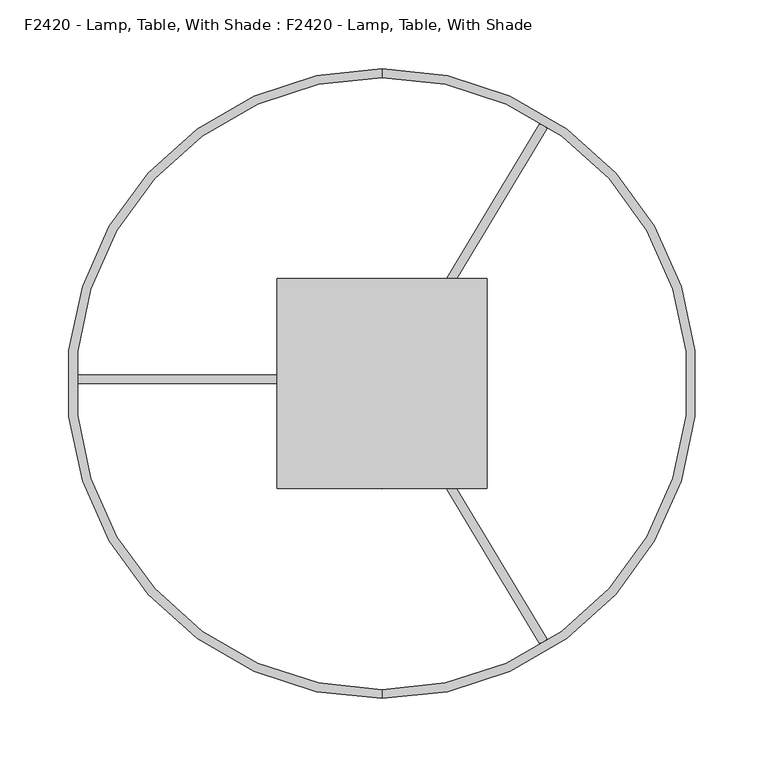
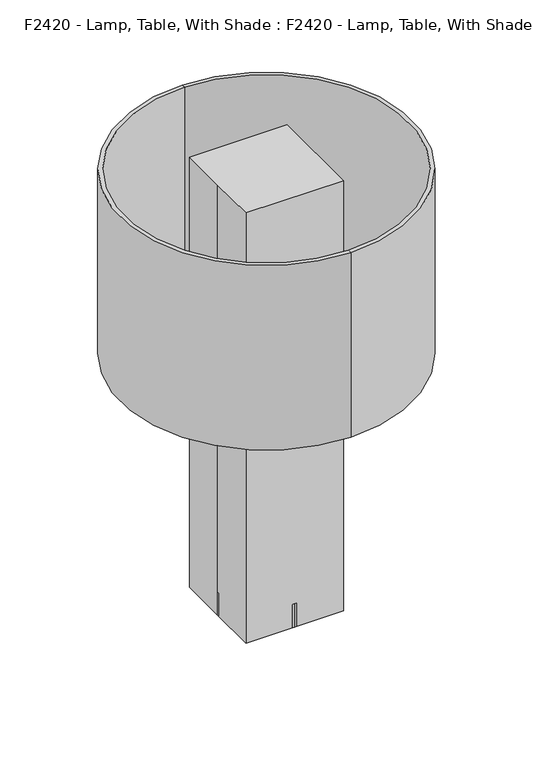
"""IFC4 building model written with IfcOpenShell, lengths in millimetres: proxy geometry, F2420 - Lamp, Table, With Shade : F2420 - Lamp, Table, With Shade."""

import ifcopenshell
import ifcopenshell.guid

model = None  # the IFC model being written
_history = None  # IfcOwnerHistory: only IFC2X3 demands one
_inside = {}  # id of a spatial element -> (the spatial element, [elements in it])
_under = {}  # id of a project, library or spatial element -> (it, [spatial elements below it])
_declared = {}  # id of a project -> (the project, [libraries it declares])
_typed = {}  # id of a type object -> (the type object, [elements of that type])
_made_of = {}  # id of a material, layer set ... -> (it, [elements and type objects made of it])


def new_model(schema):
    """Start an empty IFC model of exactly this schema.

    Asked for "IFC4X3", IfcOpenShell would pick the latest addendum, in which some entities
    have other attributes; the version numbers below select the first issue.
    IFC2X3 requires an IfcOwnerHistory on every rooted entity: one is made here for all.
    """
    global model, _history
    if schema == "IFC4X3":
        model = ifcopenshell.file(schema_version=(4, 3, 0, 0))
    else:
        model = ifcopenshell.file(schema=schema)
    _inside.clear()
    _under.clear()
    _declared.clear()
    _typed.clear()
    _made_of.clear()
    _history = None
    if model.schema == "IFC2X3":
        org = make("IfcOrganization", Name="unknown")
        user = make(
            "IfcPersonAndOrganization",
            ThePerson=make("IfcPerson", FamilyName="unknown"),
            TheOrganization=org,
        )
        app = make(
            "IfcApplication",
            ApplicationDeveloper=org,
            Version="unknown",
            ApplicationFullName="unknown",
            ApplicationIdentifier="unknown",
        )
        _history = make(
            "IfcOwnerHistory",
            OwningUser=user,
            OwningApplication=app,
            ChangeAction="ADDED",
            CreationDate=0,
        )
    return model


def make(cls, **values):
    """One entity of the class cls with the attributes given. An attribute that is None is left unset."""
    return model.create_entity(
        cls, **{name: value for name, value in values.items() if value is not None}
    )


def rooted(cls, **values):
    """An entity with a GlobalId (a new one), such as an element, a storey or a relation."""
    return make(cls, GlobalId=ifcopenshell.guid.new(), OwnerHistory=_history, **values)


def si_unit(unit_type, name, prefix=None):
    """IfcSIUnit, for example si_unit("LENGTHUNIT", "METRE", prefix="MILLI")."""
    return make("IfcSIUnit", UnitType=unit_type, Prefix=prefix, Name=name)


def assignment(units):
    """IfcUnitAssignment: the units of a project."""
    return None if units is None else make("IfcUnitAssignment", Units=units)


def point(xyz):
    """IfcCartesianPoint."""
    return None if xyz is None else make("IfcCartesianPoint", Coordinates=xyz)


def direction(xyz):
    """IfcDirection."""
    return None if xyz is None else make("IfcDirection", DirectionRatios=xyz)


def frame(location, z_axis=None, x_axis=None):
    """IfcAxis2Placement3D, a coordinate frame: its origin and axes. An axis left out is left unset."""
    return make(
        "IfcAxis2Placement3D",
        Location=point(location),
        Axis=direction(z_axis),
        RefDirection=direction(x_axis),
    )


def frame_2d(location, x_axis=None):
    """IfcAxis2Placement2D, a coordinate frame in the plane: its origin and x axis."""
    return make(
        "IfcAxis2Placement2D", Location=point(location), RefDirection=direction(x_axis)
    )


def origin():
    """The frame at (0, 0, 0) with its axes left unset."""
    return frame((0.0, 0.0, 0.0))


def origin_with_axes():
    """The frame at (0, 0, 0) with the z axis (0, 0, 1) and the x axis (1, 0, 0) written out."""
    return frame((0.0, 0.0, 0.0), z_axis=(0.0, 0.0, 1.0), x_axis=(1.0, 0.0, 0.0))


def place(relative_to, where):
    """IfcLocalPlacement: puts the frame where relative to a parent placement (None: the world)."""
    return make(
        "IfcLocalPlacement", PlacementRelTo=relative_to, RelativePlacement=where
    )


def context(
    kind, dimensions, precision=None, world=None, true_north=None, identifier=None
):
    """IfcGeometricRepresentationContext, for example the 3D "Model" context."""
    return make(
        "IfcGeometricRepresentationContext",
        ContextIdentifier=identifier,
        ContextType=kind,
        CoordinateSpaceDimension=dimensions,
        Precision=precision,
        WorldCoordinateSystem=world,
        TrueNorth=true_north,
    )


def project(units=None, contexts=None):
    """IfcProject with its units and contexts."""
    return rooted(
        "IfcProject",
        Name="project",
        RepresentationContexts=contexts,
        UnitsInContext=assignment(units),
    )


def spatial(cls, under=None, at=None, **own):
    """A site, building, storey or space (cls), placed at a placement, below another one or the project."""
    s = rooted(cls, ObjectPlacement=at, **own)
    if under is not None:
        _under.setdefault(under.id(), (under, []))[1].append(s)
    return s


def polyline(points):
    """IfcPolyline through the points."""
    return make("IfcPolyline", Points=[point(p) for p in points])


def circle_curve(where, radius):
    """IfcCircle in the frame where."""
    return make("IfcCircle", Position=where, Radius=radius)


def ellipse_curve(where, semi_axis1, semi_axis2):
    """IfcEllipse in the frame where."""
    return make(
        "IfcEllipse", Position=where, SemiAxis1=semi_axis1, SemiAxis2=semi_axis2
    )


def trimmed(basis, trim1, trim2, sense, master):
    """IfcTrimmedCurve: the piece of a basis curve between two trims."""
    return make(
        "IfcTrimmedCurve",
        BasisCurve=basis,
        Trim1=trim1,
        Trim2=trim2,
        SenseAgreement=sense,
        MasterRepresentation=master,
    )


def segment(curve, same_sense, transition):
    """IfcCompositeCurveSegment."""
    return make(
        "IfcCompositeCurveSegment",
        Transition=transition,
        SameSense=same_sense,
        ParentCurve=curve,
    )


def composite_curve(segments, self_intersect=None):
    """IfcCompositeCurve: segments joined end to end."""
    return make("IfcCompositeCurve", Segments=segments, SelfIntersect=self_intersect)


def outline(outer, holes=None, kind="AREA"):
    """IfcArbitraryClosedProfileDef: a profile drawn as a closed curve; with holes, ...WithVoids."""
    if holes is None:
        return make("IfcArbitraryClosedProfileDef", ProfileType=kind, OuterCurve=outer)
    return make(
        "IfcArbitraryProfileDefWithVoids",
        ProfileType=kind,
        OuterCurve=outer,
        InnerCurves=holes,
    )


def extrude(swept, where, along, depth):
    """IfcExtrudedAreaSolid: the profile swept, set in the frame where, extruded along a direction by depth."""
    return make(
        "IfcExtrudedAreaSolid",
        SweptArea=swept,
        Position=where,
        ExtrudedDirection=direction(along),
        Depth=depth,
    )


def shape(context_of_items, identifier, shape_type, items):
    """IfcShapeRepresentation: the items that make up one representation, for example the "Body"."""
    return make(
        "IfcShapeRepresentation",
        ContextOfItems=context_of_items,
        RepresentationIdentifier=identifier,
        RepresentationType=shape_type,
        Items=items,
    )


def source(mapping_origin, context_of_items, identifier, shape_type, items):
    """IfcRepresentationMap: a shape defined once, which mapped items show again and again."""
    return make(
        "IfcRepresentationMap",
        MappingOrigin=mapping_origin,
        MappedRepresentation=shape(context_of_items, identifier, shape_type, items),
    )


def transform(
    local_origin,
    x_axis=None,
    y_axis=None,
    z_axis=None,
    scale=None,
    scale2=None,
    scale3=None,
    uniform=True,
):
    """IfcCartesianTransformationOperator3D, or its non-uniform kind. x_axis, y_axis, z_axis: its Axis1, 2, 3."""
    if uniform:
        return make(
            "IfcCartesianTransformationOperator3D",
            Axis1=direction(x_axis),
            Axis2=direction(y_axis),
            LocalOrigin=point(local_origin),
            Scale=scale,
            Axis3=direction(z_axis),
        )
    return make(
        "IfcCartesianTransformationOperator3DnonUniform",
        Axis1=direction(x_axis),
        Axis2=direction(y_axis),
        LocalOrigin=point(local_origin),
        Scale=scale,
        Axis3=direction(z_axis),
        Scale2=scale2,
        Scale3=scale3,
    )


def mapped(mapping_source, mapping_target):
    """IfcMappedItem: shows the shape of a source again, moved by a transform."""
    return make(
        "IfcMappedItem", MappingSource=mapping_source, MappingTarget=mapping_target
    )


def made_of(thing, what):
    """Note that an element or type object is made of a material, layer set ...; save() writes the relation."""
    if what is not None:
        _made_of.setdefault(what.id(), (what, []))[1].append(thing)
    return thing


def element(
    cls,
    number,
    at=None,
    inside=None,
    cuts=None,
    type_object=None,
    material=None,
    context=None,
    identifier="Body",
    shape_type=None,
    held_by="IfcProductDefinitionShape",
    body=None,
    shapes=None,
    **own,
):
    """One element of the class cls, such as IfcWall. Its Tag is "e" and its number.

    at: its placement. inside: the storey or other place that contains it. cuts: it is an
    opening in that element (IfcRelVoidsElement). A single representation is given by context,
    identifier, shape_type and body (its items); several are given by shapes. held_by: the class
    of the entity that holds the representations. save() writes the other relations.
    """
    e = rooted(cls, Tag="e%d" % number, ObjectPlacement=at, **own)
    if body is not None:
        shapes = [shape(context, identifier, shape_type, body)]
    if shapes is not None:
        e.Representation = make(held_by, Representations=shapes)
    if inside is not None:
        _inside.setdefault(inside.id(), (inside, []))[1].append(e)
    if cuts is not None:
        rooted(
            "IfcRelVoidsElement", RelatingBuildingElement=cuts, RelatedOpeningElement=e
        )
    if type_object is not None:
        _typed.setdefault(type_object.id(), (type_object, []))[1].append(e)
    return made_of(e, material)


def aggregate(whole, parts):
    """IfcRelAggregates: a whole, such as a stair, and the parts it consists of."""
    return rooted("IfcRelAggregates", RelatingObject=whole, RelatedObjects=parts)


def save(model, path):
    """Write the relations noted so far, then the file.

    IfcRelAggregates (storeys below a building ...), IfcRelContainedInSpatialStructure (elements
    in a storey), IfcRelDefinesByType, IfcRelAssociatesMaterial and IfcRelDeclares: one each for
    every whole, place, type object, material and project.
    """
    for whole, parts in _under.values():
        aggregate(whole, parts)
    for where, things in _inside.values():
        rooted(
            "IfcRelContainedInSpatialStructure",
            RelatedElements=things,
            RelatingStructure=where,
        )
    for kind, things in _typed.values():
        rooted("IfcRelDefinesByType", RelatedObjects=things, RelatingType=kind)
    for what, things in _made_of.values():
        rooted("IfcRelAssociatesMaterial", RelatedObjects=things, RelatingMaterial=what)
    for by, libraries in _declared.values():
        rooted("IfcRelDeclares", RelatingContext=by, RelatedDefinitions=libraries)
    model.write(path)


def plane_surface(at):
    """IfcPlane: the flat surface through the origin of the frame at, square to its z axis."""
    return make("IfcPlane", Position=at)


def cylinder_surface(at, radius):
    """IfcCylindricalSurface: all points at the distance radius from the z axis of the frame at."""
    return make("IfcCylindricalSurface", Position=at, Radius=radius)


def revolved_surface(curve, axis_point, axis_direction):
    """IfcSurfaceOfRevolution: the curve turned about the line through axis_point along axis_direction."""
    return make(
        "IfcSurfaceOfRevolution",
        SweptCurve=make("IfcArbitraryOpenProfileDef", ProfileType="CURVE", Curve=curve),
        AxisPosition=make("IfcAxis1Placement", Location=point(axis_point), Axis=direction(axis_direction)),
    )


def advanced_brep(points, edges, surfaces, faces):
    """IfcAdvancedBrep: a solid bounded by faces that lie on surfaces and meet in shared edges.

    An edge is (start, end): straight between two places in points (the first is 0);
    or (start, end, curve); or (start, end, curve, False) where it runs against its curve.
    A face is (place in surfaces, loops), or (place, loops, False) where it looks against
    its surface's normal. A loop lists edges by number (the first is 1), with a minus sign
    where the edge is run from its end to its start. The first loop is the outer one.
    """
    corners = [point(p) for p in points]
    vertices = [make("IfcVertexPoint", VertexGeometry=c) for c in corners]
    made = []
    for start, end, *more in edges:
        made.append(
            make(
                "IfcEdgeCurve",
                EdgeStart=vertices[start],
                EdgeEnd=vertices[end],
                EdgeGeometry=more[0] if more else make("IfcPolyline", Points=[corners[start], corners[end]]),
                SameSense=more[1] if len(more) > 1 else True,
            )
        )
    hull = []
    for where, loops, *sense in faces:
        bounds = []
        for j, loop in enumerate(loops):
            ring = [make("IfcOrientedEdge", EdgeElement=made[abs(k) - 1], Orientation=k > 0) for k in loop]
            bounds.append(
                make(
                    "IfcFaceOuterBound" if j == 0 else "IfcFaceBound",
                    Bound=make("IfcEdgeLoop", EdgeList=ring),
                    Orientation=True,
                )
            )
        hull.append(make("IfcAdvancedFace", Bounds=bounds, FaceSurface=surfaces[where], SameSense=sense[0] if sense else True))
    return make("IfcAdvancedBrep", Outer=make("IfcClosedShell", CfsFaces=hull))


def f2420_lamp_table_with_shade_f2420_lamp_table_with_shade_198ff228(model_context):
    return source(origin(), model_context, "Body", "SolidModel", [
        extrude(outline(composite_curve([segment(trimmed(circle_curve(frame_2d((112.7651926, 179.9675314)), 8.6265279), [point((114.1748041, 188.4781117))], [point((119.6178165, 185.2076199))], False, "CARTESIAN"), True, "CONTINUOUS"), segment(polyline([(119.6178165, 185.2076199), (18.3833354, 16.7251502)]), True, "CONTINUOUS"), segment(trimmed(circle_curve(frame_2d((6.6305332, 9.5999352)), 13.7439822), [point((18.3833354, 16.7251502))], [point((13.7557482, 21.3527373))], True, "CARTESIAN"), True, "CONTINUOUS"), segment(polyline([(13.7557482, 21.3527373), (114.1748041, 188.4781117)]), True, "CONTINUOUS")], self_intersect=False)), frame((0.0, 0.0, 546.1), z_axis=(0.0, 0.0, 1.0), x_axis=(1.0, 0.0, 0.0)), (0.0, 0.0, 1.0), 6.35),
        extrude(outline(composite_curve([segment(polyline([(114.1748041, -188.4781117), (13.7557482, -21.3527373)]), True, "CONTINUOUS"), segment(trimmed(circle_curve(frame_2d((6.6305332, -9.5999352)), 13.7439822), [point((13.7557482, -21.3527373))], [point((18.3833354, -16.7251502))], True, "CARTESIAN"), True, "CONTINUOUS"), segment(polyline([(18.3833354, -16.7251502), (119.6178165, -185.2076199)]), True, "CONTINUOUS"), segment(trimmed(circle_curve(frame_2d((112.7651926, -179.9675314)), 8.6265279), [point((119.6178165, -185.2076199))], [point((114.1748041, -188.4781117))], False, "CARTESIAN"), True, "CONTINUOUS")], self_intersect=False)), frame((0.0, 0.0, 546.1), z_axis=(0.0, 0.0, 1.0), x_axis=(1.0, 0.0, 0.0)), (0.0, 0.0, 1.0), 6.35),
        extrude(outline(composite_curve([segment(trimmed(circle_curve(frame_2d((-217.8006717, 2.2107608)), 4.9682981), [point((-222.25, 0.0))], [point((-220.5485226, 6.35))], False, "CARTESIAN"), True, "CONTINUOUS"), segment(polyline([(-220.5485226, 6.35), (-24.5934442, 6.35)]), True, "CONTINUOUS"), segment(trimmed(circle_curve(frame_2d((-15.109772, 3.175)), 10.0010332), [point((-24.5934442, 6.35))], [point((-24.5934442, 0.0))], True, "CARTESIAN"), True, "CONTINUOUS"), segment(polyline([(-24.5934442, 0.0), (-222.25, 0.0)]), True, "CONTINUOUS")], self_intersect=False)), frame((0.0, 0.0, 546.1), z_axis=(0.0, 0.0, 1.0), x_axis=(1.0, 0.0, 0.0)), (0.0, 0.0, 1.0), 6.35),
        advanced_brep(
        [(0.0, 76.2, 38.1), (0.0, 76.2, 0.0), (0.0, -76.2, 0.0), (0.0, -76.2, 38.1), (0.0, 38.1, 38.1), (0.0, -38.1, 38.1), (0.0, 38.1, 342.9), (0.0, -38.1, 342.9), (0.0, 25.4, 342.9), (0.0, -25.4, 342.9), (0.0, 25.4, 566.3974415), (0.0, -25.4, 566.3974415), (0.0, 0.0, 566.3974415), (0.0, 0.0, 0.0)],
        [
            (0, 1),
            (1, 2, circle_curve(frame((0.0, 0.0, 0.0), z_axis=(0.0, 0.0, 1.0), x_axis=(0.0, -1.0, 0.0)), 76.2)),
            (2, 3),
            (3, 0, circle_curve(frame((0.0, 0.0, 38.1), z_axis=(0.0, 0.0, -1.0), x_axis=(0.0, -1.0, 0.0)), 76.2)),
            (2, 1, circle_curve(frame((0.0, 0.0, 0.0), z_axis=(0.0, 0.0, 1.0), x_axis=(0.0, -1.0, 0.0)), 76.2)),
            (0, 3, circle_curve(frame((0.0, 0.0, 38.1), z_axis=(0.0, 0.0, -1.0), x_axis=(0.0, -1.0, 0.0)), 76.2)),
            (4, 0),
            (3, 5),
            (5, 4, circle_curve(frame((0.0, 0.0, 38.1), z_axis=(0.0, 0.0, -1.0), x_axis=(0.0, -1.0, 0.0)), 38.1)),
            (4, 5, circle_curve(frame((0.0, 0.0, 38.1), z_axis=(0.0, 0.0, -1.0), x_axis=(0.0, -1.0, 0.0)), 38.1)),
            (6, 4, circle_curve(frame((0.0, -531.1639762, 190.5), z_axis=(-1.0, 0.0, 0.0), x_axis=(0.0, 1.0, 0.0)), 589.3108132)),
            (5, 7, circle_curve(frame((0.0, 531.1639762, 190.5), z_axis=(-1.0, 0.0, 0.0), x_axis=(0.0, -1.0, 0.0)), 589.3108132)),
            (7, 6, circle_curve(frame((0.0, 0.0, 342.9), z_axis=(0.0, 0.0, -1.0), x_axis=(0.0, -1.0, 0.0)), 38.1)),
            (6, 7, circle_curve(frame((0.0, 0.0, 342.9), z_axis=(0.0, 0.0, -1.0), x_axis=(0.0, -1.0, 0.0)), 38.1)),
            (8, 6),
            (7, 9),
            (9, 8, circle_curve(frame((0.0, 0.0, 342.9), z_axis=(0.0, 0.0, -1.0), x_axis=(0.0, -1.0, 0.0)), 25.4)),
            (8, 9, circle_curve(frame((0.0, 0.0, 342.9), z_axis=(0.0, 0.0, -1.0), x_axis=(0.0, -1.0, 0.0)), 25.4)),
            (10, 8),
            (9, 11),
            (11, 10, circle_curve(frame((0.0, 0.0, 566.3974415), z_axis=(0.0, 0.0, -1.0), x_axis=(0.0, -1.0, 0.0)), 25.4)),
            (10, 11, circle_curve(frame((0.0, 0.0, 566.3974415), z_axis=(0.0, 0.0, -1.0), x_axis=(0.0, -1.0, 0.0)), 25.4)),
            (12, 10),
            (11, 12),
            (1, 13),
            (13, 2),
        ],
        [
            cylinder_surface(frame((0.0, 0.0, 469.9), z_axis=(0.0, 0.0, 1.0), x_axis=(0.0, -1.0, 0.0)), 76.2),
            plane_surface(frame((0.0, 0.0, 38.1), z_axis=(0.0, 0.0, 1.0), x_axis=(0.0, -1.0, 0.0))),
            revolved_surface(trimmed(ellipse_curve(frame((0.0, 531.1639762, 190.5), z_axis=(-1.0, 0.0, 0.0), x_axis=(0.0, -1.0, 0.0)), 589.3108132, 589.3108132), [point((0.0, -38.1, 38.1))], [point((0.0, -38.1, 342.9))], True, "CARTESIAN"), (0.0, 0.0, 469.9), (0.0, 0.0, 1.0)),
            plane_surface(frame((0.0, 0.0, 342.9), z_axis=(0.0, 0.0, 1.0), x_axis=(0.0, -1.0, 0.0))),
            cylinder_surface(frame((0.0, 0.0, 469.9), z_axis=(0.0, 0.0, 1.0), x_axis=(0.0, -1.0, 0.0)), 25.4),
            plane_surface(frame((0.0, 0.0, 566.3974415), z_axis=(0.0, 0.0, 1.0), x_axis=(0.0, -1.0, 0.0))),
            plane_surface(frame((0.0, 0.0, 0.0), z_axis=(0.0, 0.0, -1.0), x_axis=(0.0, -1.0, 0.0))),
        ],
        [
            (0, [[1, 2, 3, 4]]),
            (0, [[-3, 5, -1, 6]]),
            (1, [[7, -4, 8, 9]]),
            (1, [[-8, -6, -7, 10]]),
            (2, [[11, -9, 12, 13]]),
            (2, [[-12, -10, -11, 14]]),
            (3, [[15, -13, 16, 17]]),
            (3, [[-16, -14, -15, 18]]),
            (4, [[19, -17, 20, 21]]),
            (4, [[-20, -18, -19, 22]]),
            (5, [[23, -21, 24]]),
            (5, [[-24, -22, -23]]),
            (6, [[25, 26, -2]]),
            (6, [[-26, -25, -5]]),
        ],
    ),
        advanced_brep(
        [(0.0, 222.25, 406.4), (0.0, 222.25, 711.2), (0.0, -222.25, 711.2), (0.0, -222.25, 406.4), (0.0, 228.6, 406.4), (0.0, -228.6, 406.4), (0.0, 228.6, 711.2), (0.0, -228.6, 711.2)],
        [
            (0, 1),
            (1, 2, circle_curve(frame((0.0, 0.0, 711.2), z_axis=(0.0, 0.0, 1.0), x_axis=(0.0, -1.0, 0.0)), 222.25)),
            (2, 3),
            (3, 0, circle_curve(frame((0.0, 0.0, 406.4), z_axis=(0.0, 0.0, -1.0), x_axis=(0.0, -1.0, 0.0)), 222.25)),
            (2, 1, circle_curve(frame((0.0, 0.0, 711.2), z_axis=(0.0, 0.0, 1.0), x_axis=(0.0, -1.0, 0.0)), 222.25)),
            (0, 3, circle_curve(frame((0.0, 0.0, 406.4), z_axis=(0.0, 0.0, -1.0), x_axis=(0.0, -1.0, 0.0)), 222.25)),
            (4, 0),
            (3, 5),
            (5, 4, circle_curve(frame((0.0, 0.0, 406.4), z_axis=(0.0, 0.0, -1.0), x_axis=(0.0, -1.0, 0.0)), 228.6)),
            (4, 5, circle_curve(frame((0.0, 0.0, 406.4), z_axis=(0.0, 0.0, -1.0), x_axis=(0.0, -1.0, 0.0)), 228.6)),
            (6, 4),
            (5, 7),
            (7, 6, circle_curve(frame((0.0, 0.0, 711.2), z_axis=(0.0, 0.0, -1.0), x_axis=(0.0, -1.0, 0.0)), 228.6)),
            (6, 7, circle_curve(frame((0.0, 0.0, 711.2), z_axis=(0.0, 0.0, -1.0), x_axis=(0.0, -1.0, 0.0)), 228.6)),
            (1, 6),
            (7, 2),
        ],
        [
            revolved_surface(polyline([(0.0, -222.25, 711.2), (0.0, -222.25, 406.4)]), (0.0, 0.0, 711.2), (0.0, 0.0, 1.0)),
            plane_surface(frame((0.0, 0.0, 406.4), z_axis=(0.0, 0.0, -1.0), x_axis=(0.0, -1.0, 0.0))),
            cylinder_surface(frame((0.0, 0.0, 711.2), z_axis=(0.0, 0.0, 1.0), x_axis=(0.0, -1.0, 0.0)), 228.6),
            plane_surface(frame((0.0, 0.0, 711.2), z_axis=(0.0, 0.0, 1.0), x_axis=(0.0, -1.0, 0.0))),
        ],
        [
            (0, [[1, 2, 3, 4]]),
            (0, [[-3, 5, -1, 6]]),
            (1, [[7, -4, 8, 9]]),
            (1, [[-8, -6, -7, 10]]),
            (2, [[11, -9, 12, 13]]),
            (2, [[-12, -10, -11, 14]]),
            (3, [[15, -13, 16, -2]]),
            (3, [[-16, -14, -15, -5]]),
        ],
    ),
        extrude(outline(polyline([(-76.2, -76.2), (-76.2, 0.0), (-76.2, 76.2), (76.2, 76.2), (76.2, -76.2), (-76.2, -76.2)])), origin_with_axes(), (0.0, 0.0, 1.0), 711.2),
    ])


if __name__ == "__main__":
    model = new_model("IFC4")
    model_context = context("Model", 3, world=origin())
    ifc_project = project(units=[si_unit("LENGTHUNIT", "METRE", prefix="MILLI")], contexts=[model_context])
    site = spatial("IfcSite", under=ifc_project)
    building = spatial("IfcBuilding", under=site)
    placement = place(None, origin())
    f2420_lamp_table_with_shade_f2420_lamp_table_with_shade_shape = f2420_lamp_table_with_shade_f2420_lamp_table_with_shade_198ff228(model_context)
    element("IfcBuildingElementProxy", 1, Name="F2420 - Lamp, Table, With Shade : F2420 - Lamp, Table, With Shade", ObjectType="F2420 - Lamp, Table, With Shade : F2420 - Lamp, Table, With Shade", at=placement, inside=building, context=model_context, shape_type="MappedRepresentation", body=[
        mapped(f2420_lamp_table_with_shade_f2420_lamp_table_with_shade_shape, transform((0.0, 0.0, 0.0), x_axis=(1.0, 0.0, 0.0), y_axis=(0.0, 1.0, 0.0), z_axis=(0.0, 0.0, 1.0))),
    ])
    save(model, "model.ifc")

# Revit data of these elements
# Project information
#   Sheets - Total = "6"
#   Project Issue Date = "Issue Date"
#   Project Status = "Project Status"
#   Client Name = "Owner"
#   Project Address = "Enter address here"
#   Project Name = "Project Name"
#   Project Number = "Project Number"
#   Publication Date = "30-Jan-15"
# Type "F2420 - Lamp, Table, With Shade : F2420 - Lamp, Table, With Shade"
#   Watts2 = "0"
#   Watts1 = "120"
#   Unit_Issue = "EA"
#   UTIL_6_Misc = "-"
#   UTIL_5_NonMedGas = "-"
#   UTIL_4_MiscGas = "-"
#   UTIL_3_MedGas = "-"
#   UTIL_2_Elec = "A"
#   UTIL_1_WaterDrain = "-"
#   Nomenclature = "Lamp, Table, With Shade"
#   NSN = "6230"
#   Location [instance default] = ""
#   JSN = "F2420"
#   Fund_Source_VA = "-"
#   Fund_Source_Navy = "-"
#   Fund_Source_Army = "-"
#   Fund_Source_AF = "-"
#   ELEC_Volts2 = "0"
#   ELEC_Volts1 = "120"
#   ELEC_Phase2 = "0"
#   ELEC_Phase1 = "1"
#   ELEC_HertzSwitch = "0"
#   ELEC_HertzDependent = "0"
#   ELEC_Hertz = "60"
#   ELEC_Amps2 = "0"
#   ELEC_Amps1 = "1"
#   DetailDescription = "Table lamp, 27-34\" high X 6\" wide X 6\" deep with linen shade. Convenience outlet required at point of use."
#   CAT_VA = "C"
#   CAT_Navy = "C"
#   CAT_IHS = "-"
#   CAT_Army = "C"
#   CAT_AF = "C"
#   BTUperhour = "0"
#   Weight_IP = 14
#   DIM_Width_IP = 0' - 6"
#   DIM_Height_IP = 2' - 4"
#   DIM_Depth_IP = 0' - 6"
# Element 1 (IfcBuildingElementProxy, "F2420 - Lamp, Table, With Shade : F2420 - Lamp, Table, With Shade")
#   Location = "DUTY1"
#   Materials on its faces: "EquipSpace"
# Materials
#   "EquipSpace": class "Unassigned", colour RGB 221 217 195, transparency 0.5
